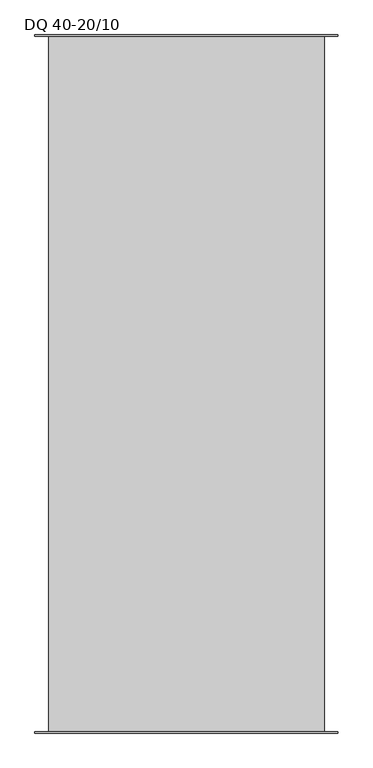
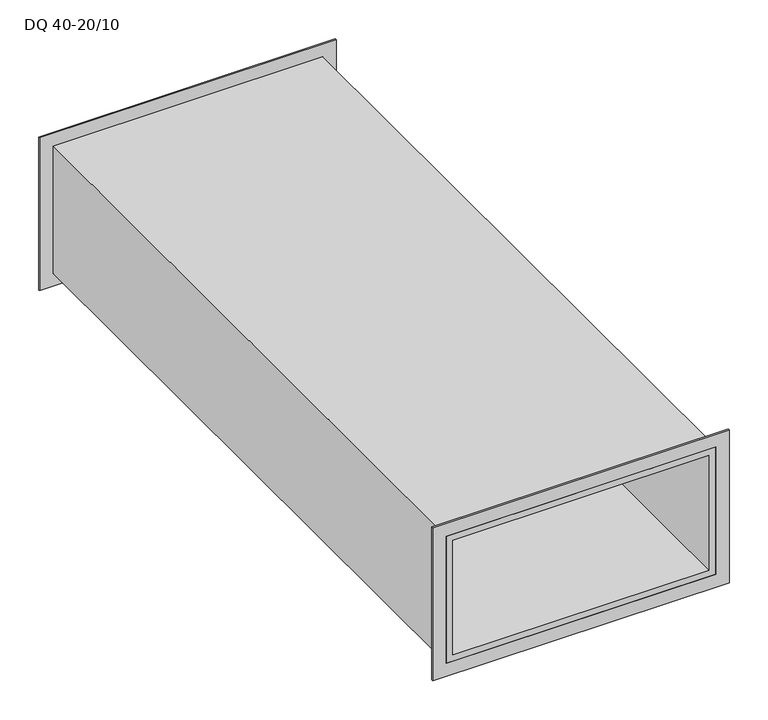
"""IFC4 building model written with IfcOpenShell, lengths in millimetres: proxy geometry, Шумоглушитель пластинчатый DQ : DQ 40-20/10."""

from ifc_helpers import new_model, si_unit, frame, origin, place, context, project, spatial, polyline, outline, extrude, source, transform, mapped, element, save


def dq_40_20_10_5c174b56(model_context):
    return source(origin(), model_context, "Body", "SweptSolid", [
        extrude(outline(polyline([(120.0, 220.0), (120.0, -220.0), (-120.0, -220.0), (-120.0, 220.0), (120.0, 220.0)]), holes=[polyline([(-100.0, 200.0), (-100.0, -200.0), (100.0, -200.0), (100.0, 200.0), (-100.0, 200.0)])]), frame((0.0, 504.0, 0.0), z_axis=(0.0, 1.0, 0.0), x_axis=(0.0, 0.0, 1.0)), (0.0, 0.0, 1.0), 2.0),
        extrude(outline(polyline([(120.0, -220.0), (-120.0, -220.0), (-120.0, 220.0), (120.0, 220.0), (120.0, -220.0)]), holes=[polyline([(100.0, 200.0), (-100.0, 200.0), (-100.0, -200.0), (100.0, -200.0), (100.0, 200.0)])]), frame((0.0, -506.0, 0.0), z_axis=(0.0, 1.0, 0.0), x_axis=(0.0, 0.0, 1.0)), (0.0, 0.0, 1.0), 2.0),
        extrude(outline(polyline([(100.0, 200.0), (100.0, -200.0), (-100.0, -200.0), (-100.0, 200.0), (100.0, 200.0)]), holes=[polyline([(90.0, 190.0), (-90.0, 190.0), (-90.0, -190.0), (90.0, -190.0), (90.0, 190.0)])]), frame((0.0, -506.0, 0.0), z_axis=(0.0, 1.0, 0.0), x_axis=(0.0, 0.0, 1.0)), (0.0, 0.0, 1.0), 1012.0),
    ])


if __name__ == "__main__":
    model = new_model("IFC4")
    model_context = context("Model", 3, world=origin())
    ifc_project = project(units=[si_unit("LENGTHUNIT", "METRE", prefix="MILLI")], contexts=[model_context])
    site = spatial("IfcSite", under=ifc_project)
    building = spatial("IfcBuilding", under=site)
    placement = place(None, origin())
    dq_40_20_10_shape = dq_40_20_10_5c174b56(model_context)
    element("IfcBuildingElementProxy", 1, Name="Шумоглушитель пластинчатый DQ : DQ 40-20/10", ObjectType="Шумоглушитель пластинчатый DQ : DQ 40-20/10", at=placement, inside=building, context=model_context, shape_type="MappedRepresentation", body=[
        mapped(dq_40_20_10_shape, transform((0.0, 0.0, 0.0), x_axis=(1.0, 0.0, 0.0), y_axis=(0.0, 1.0, 0.0), z_axis=(0.0, 0.0, 1.0))),
    ])
    save(model, "model.ifc")

# Revit data of these elements
# Type "Шумоглушитель пластинчатый DQ : DQ 40-20/10"
#   Manufacturer = "WAER"
#   URL = "https://waer-air.com/"
#   ADSK_Система_Имя [instance default] = ""
#   ADSK_Наименование краткое = "DQ 40-20/10"
#   ADSK_Наименование = "Шумоглушитель пластинчатый DQ 40-20/10"
#   ADSK_Масса_Текст = "26.1"
#   ADSK_Марка = ""
#   ADSK_Код изделия = ""
#   ADSK_Завод-изготовитель = "WAER"
#   ADSK_Единица измерения = "шт."
#   ADSK_Расход воздуха = 0 m³/h
#   ADSK_Размер_Ширина = 400 mm
#   ADSK_Размер_Длина = 1012 mm
#   ADSK_Размер_Высота = 200 mm
#   ADSK_Потеря давления воздуха = 0.0 Pa
#   ADSK_Масса = 26.1
#   ADSK_Количество = 1
#   Default Elevation = 0
#   Keynote = ""
